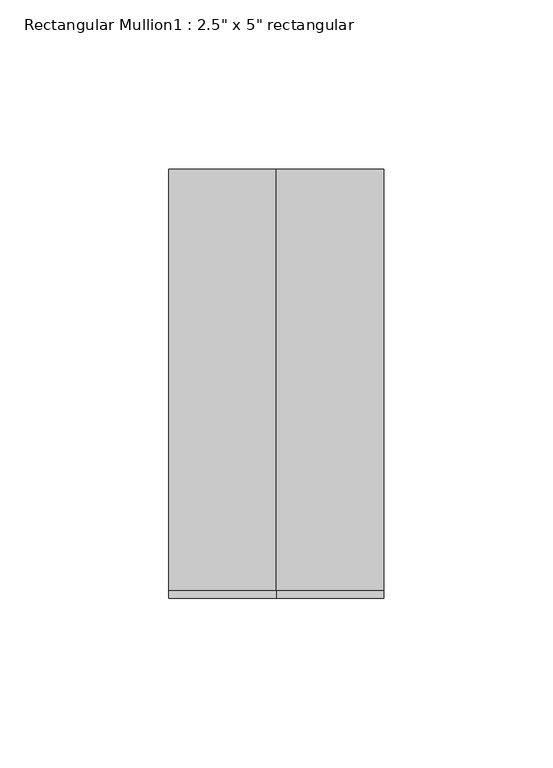
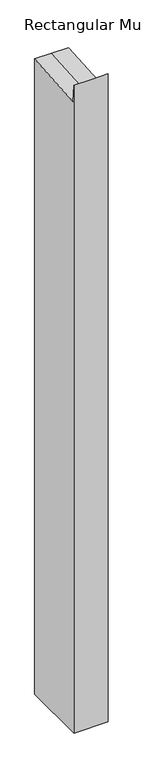
"""IFC4 building model written with IfcOpenShell, lengths in millimetres: member geometry."""

import ifcopenshell
import ifcopenshell.guid

model = None  # the IFC model being written
_history = None  # IfcOwnerHistory: only IFC2X3 demands one
_inside = {}  # id of a spatial element -> (the spatial element, [elements in it])
_under = {}  # id of a project, library or spatial element -> (it, [spatial elements below it])
_declared = {}  # id of a project -> (the project, [libraries it declares])
_typed = {}  # id of a type object -> (the type object, [elements of that type])
_made_of = {}  # id of a material, layer set ... -> (it, [elements and type objects made of it])


def new_model(schema):
    """Start an empty IFC model of exactly this schema.

    Asked for "IFC4X3", IfcOpenShell would pick the latest addendum, in which some entities
    have other attributes; the version numbers below select the first issue.
    IFC2X3 requires an IfcOwnerHistory on every rooted entity: one is made here for all.
    """
    global model, _history
    if schema == "IFC4X3":
        model = ifcopenshell.file(schema_version=(4, 3, 0, 0))
    else:
        model = ifcopenshell.file(schema=schema)
    _inside.clear()
    _under.clear()
    _declared.clear()
    _typed.clear()
    _made_of.clear()
    _history = None
    if model.schema == "IFC2X3":
        org = make("IfcOrganization", Name="unknown")
        user = make(
            "IfcPersonAndOrganization",
            ThePerson=make("IfcPerson", FamilyName="unknown"),
            TheOrganization=org,
        )
        app = make(
            "IfcApplication",
            ApplicationDeveloper=org,
            Version="unknown",
            ApplicationFullName="unknown",
            ApplicationIdentifier="unknown",
        )
        _history = make(
            "IfcOwnerHistory",
            OwningUser=user,
            OwningApplication=app,
            ChangeAction="ADDED",
            CreationDate=0,
        )
    return model


def make(cls, **values):
    """One entity of the class cls with the attributes given. An attribute that is None is left unset."""
    return model.create_entity(
        cls, **{name: value for name, value in values.items() if value is not None}
    )


def rooted(cls, **values):
    """An entity with a GlobalId (a new one), such as an element, a storey or a relation."""
    return make(cls, GlobalId=ifcopenshell.guid.new(), OwnerHistory=_history, **values)


def si_unit(unit_type, name, prefix=None):
    """IfcSIUnit, for example si_unit("LENGTHUNIT", "METRE", prefix="MILLI")."""
    return make("IfcSIUnit", UnitType=unit_type, Prefix=prefix, Name=name)


def assignment(units):
    """IfcUnitAssignment: the units of a project."""
    return None if units is None else make("IfcUnitAssignment", Units=units)


def point(xyz):
    """IfcCartesianPoint."""
    return None if xyz is None else make("IfcCartesianPoint", Coordinates=xyz)


def direction(xyz):
    """IfcDirection."""
    return None if xyz is None else make("IfcDirection", DirectionRatios=xyz)


def frame(location, z_axis=None, x_axis=None):
    """IfcAxis2Placement3D, a coordinate frame: its origin and axes. An axis left out is left unset."""
    return make(
        "IfcAxis2Placement3D",
        Location=point(location),
        Axis=direction(z_axis),
        RefDirection=direction(x_axis),
    )


def origin():
    """The frame at (0, 0, 0) with its axes left unset."""
    return frame((0.0, 0.0, 0.0))


def place(relative_to, where):
    """IfcLocalPlacement: puts the frame where relative to a parent placement (None: the world)."""
    return make(
        "IfcLocalPlacement", PlacementRelTo=relative_to, RelativePlacement=where
    )


def context(
    kind, dimensions, precision=None, world=None, true_north=None, identifier=None
):
    """IfcGeometricRepresentationContext, for example the 3D "Model" context."""
    return make(
        "IfcGeometricRepresentationContext",
        ContextIdentifier=identifier,
        ContextType=kind,
        CoordinateSpaceDimension=dimensions,
        Precision=precision,
        WorldCoordinateSystem=world,
        TrueNorth=true_north,
    )


def project(units=None, contexts=None):
    """IfcProject with its units and contexts."""
    return rooted(
        "IfcProject",
        Name="project",
        RepresentationContexts=contexts,
        UnitsInContext=assignment(units),
    )


def spatial(cls, under=None, at=None, **own):
    """A site, building, storey or space (cls), placed at a placement, below another one or the project."""
    s = rooted(cls, ObjectPlacement=at, **own)
    if under is not None:
        _under.setdefault(under.id(), (under, []))[1].append(s)
    return s


def faces_of(points, faces, orient=None, outer=None):
    """IfcFace entities. A face is a list of loops; a loop is a list of indices into points, from 0.

    orient and outer hold one flag for each loop. By default every Orientation is true, the
    first loop of a face is its IfcFaceOuterBound and the others are IfcFaceBound.
    """
    made = []
    for i, loops in enumerate(faces):
        bounds = []
        for j, loop in enumerate(loops):
            is_outer = j == 0 if outer is None else outer[i][j]
            bounds.append(
                make(
                    "IfcFaceOuterBound" if is_outer else "IfcFaceBound",
                    Bound=make("IfcPolyLoop", Polygon=[points[k] for k in loop]),
                    Orientation=True if orient is None else orient[i][j],
                )
            )
        made.append(make("IfcFace", Bounds=bounds))
    return made


def faceted_brep(points, faces, orient=None, outer=None, voids=None):
    """IfcFacetedBrep: a solid bounded by flat faces; with voids (closed shells), ...WithVoids."""
    shared = [point(p) for p in points]
    hull = make("IfcClosedShell", CfsFaces=faces_of(shared, faces, orient, outer))
    if voids is None:
        return make("IfcFacetedBrep", Outer=hull)
    return make(
        "IfcFacetedBrepWithVoids",
        Outer=hull,
        Voids=[
            make(cls, CfsFaces=faces_of(shared, fs, o, b)) for cls, fs, o, b in voids
        ],
    )


def shape(context_of_items, identifier, shape_type, items):
    """IfcShapeRepresentation: the items that make up one representation, for example the "Body"."""
    return make(
        "IfcShapeRepresentation",
        ContextOfItems=context_of_items,
        RepresentationIdentifier=identifier,
        RepresentationType=shape_type,
        Items=items,
    )


def source(mapping_origin, context_of_items, identifier, shape_type, items):
    """IfcRepresentationMap: a shape defined once, which mapped items show again and again."""
    return make(
        "IfcRepresentationMap",
        MappingOrigin=mapping_origin,
        MappedRepresentation=shape(context_of_items, identifier, shape_type, items),
    )


def transform(
    local_origin,
    x_axis=None,
    y_axis=None,
    z_axis=None,
    scale=None,
    scale2=None,
    scale3=None,
    uniform=True,
):
    """IfcCartesianTransformationOperator3D, or its non-uniform kind. x_axis, y_axis, z_axis: its Axis1, 2, 3."""
    if uniform:
        return make(
            "IfcCartesianTransformationOperator3D",
            Axis1=direction(x_axis),
            Axis2=direction(y_axis),
            LocalOrigin=point(local_origin),
            Scale=scale,
            Axis3=direction(z_axis),
        )
    return make(
        "IfcCartesianTransformationOperator3DnonUniform",
        Axis1=direction(x_axis),
        Axis2=direction(y_axis),
        LocalOrigin=point(local_origin),
        Scale=scale,
        Axis3=direction(z_axis),
        Scale2=scale2,
        Scale3=scale3,
    )


def mapped(mapping_source, mapping_target):
    """IfcMappedItem: shows the shape of a source again, moved by a transform."""
    return make(
        "IfcMappedItem", MappingSource=mapping_source, MappingTarget=mapping_target
    )


def made_of(thing, what):
    """Note that an element or type object is made of a material, layer set ...; save() writes the relation."""
    if what is not None:
        _made_of.setdefault(what.id(), (what, []))[1].append(thing)
    return thing


def element(
    cls,
    number,
    at=None,
    inside=None,
    cuts=None,
    type_object=None,
    material=None,
    context=None,
    identifier="Body",
    shape_type=None,
    held_by="IfcProductDefinitionShape",
    body=None,
    shapes=None,
    **own,
):
    """One element of the class cls, such as IfcWall. Its Tag is "e" and its number.

    at: its placement. inside: the storey or other place that contains it. cuts: it is an
    opening in that element (IfcRelVoidsElement). A single representation is given by context,
    identifier, shape_type and body (its items); several are given by shapes. held_by: the class
    of the entity that holds the representations. save() writes the other relations.
    """
    e = rooted(cls, Tag="e%d" % number, ObjectPlacement=at, **own)
    if body is not None:
        shapes = [shape(context, identifier, shape_type, body)]
    if shapes is not None:
        e.Representation = make(held_by, Representations=shapes)
    if inside is not None:
        _inside.setdefault(inside.id(), (inside, []))[1].append(e)
    if cuts is not None:
        rooted(
            "IfcRelVoidsElement", RelatingBuildingElement=cuts, RelatedOpeningElement=e
        )
    if type_object is not None:
        _typed.setdefault(type_object.id(), (type_object, []))[1].append(e)
    return made_of(e, material)


def aggregate(whole, parts):
    """IfcRelAggregates: a whole, such as a stair, and the parts it consists of."""
    return rooted("IfcRelAggregates", RelatingObject=whole, RelatedObjects=parts)


def save(model, path):
    """Write the relations noted so far, then the file.

    IfcRelAggregates (storeys below a building ...), IfcRelContainedInSpatialStructure (elements
    in a storey), IfcRelDefinesByType, IfcRelAssociatesMaterial and IfcRelDeclares: one each for
    every whole, place, type object, material and project.
    """
    for whole, parts in _under.values():
        aggregate(whole, parts)
    for where, things in _inside.values():
        rooted(
            "IfcRelContainedInSpatialStructure",
            RelatedElements=things,
            RelatingStructure=where,
        )
    for kind, things in _typed.values():
        rooted("IfcRelDefinesByType", RelatedObjects=things, RelatingType=kind)
    for what, things in _made_of.values():
        rooted("IfcRelAssociatesMaterial", RelatedObjects=things, RelatingMaterial=what)
    for by, libraries in _declared.values():
        rooted("IfcRelDeclares", RelatingContext=by, RelatedDefinitions=libraries)
    model.write(path)


def member_92e61aeb(model_context):
    return source(origin(), model_context, "Body", "Brep", [
        faceted_brep([(31.75, 63.5, -1249.2609667), (31.75, -63.5, -1249.2609667), (-31.75, -63.5, -1249.2609667), (-31.75, 63.5, -1249.2609667), (-31.75, 63.5, 4.3258089), (0.0, 63.5, 4.3258089), (31.75, 63.5, 4.3258089), (-31.75, -63.5, 29.5516342), (-31.75, -61.1522336, -4.315452), (31.75, -63.5, 29.5516342), (0.0, -63.5, 29.5516342), (31.75, -61.1522336, -4.315452), (0.0, -61.1522336, -4.315452)], [[[0, 1, 2, 3]], [[4, 5, 6, 0, 3]], [[7, 8, 4, 3, 2]], [[9, 10, 7, 2, 1]], [[6, 11, 9, 1, 0]], [[6, 5, 12, 11]], [[5, 4, 8, 12]], [[8, 7, 10, 12]], [[10, 9, 11, 12]]]),
    ])


if __name__ == "__main__":
    model = new_model("IFC4")
    model_context = context("Model", 3, world=origin())
    ifc_project = project(units=[si_unit("LENGTHUNIT", "METRE", prefix="MILLI")], contexts=[model_context])
    site = spatial("IfcSite", under=ifc_project)
    building = spatial("IfcBuilding", under=site)
    placement = place(None, origin())
    member_shape = member_92e61aeb(model_context)
    element("IfcMember", 1, ObjectType="Rectangular Mullion1 : 2.5\" x 5\" rectangular", at=placement, inside=building, context=model_context, shape_type="MappedRepresentation", body=[
        mapped(member_shape, transform((0.0, 0.0, 0.0), x_axis=(1.0, 0.0, 0.0), y_axis=(0.0, 1.0, 0.0), z_axis=(0.0, 0.0, 1.0))),
    ])
    save(model, "model.ifc")

# Revit data of these elements
# Type "Rectangular Mullion1 : 2.5\" x 5\" rectangular"
#   built-in parameter 1007304 = 0.416667 (stored number, unit not read)
#   built-in parameter 1007301 = 0.104167 (stored number, unit not read)
#   built-in parameter 1007300 = 0.104167 (stored number, unit not read)
# Element 1 (IfcMember, "Rectangular Mullion1 : 2.5\" x 5\" rectangular")
#   Materials on its faces: "support-frame"
# Materials
#   "support-frame": class "Unassigned", colour RGB 233 233 233, transparency 0, Cost = 0
